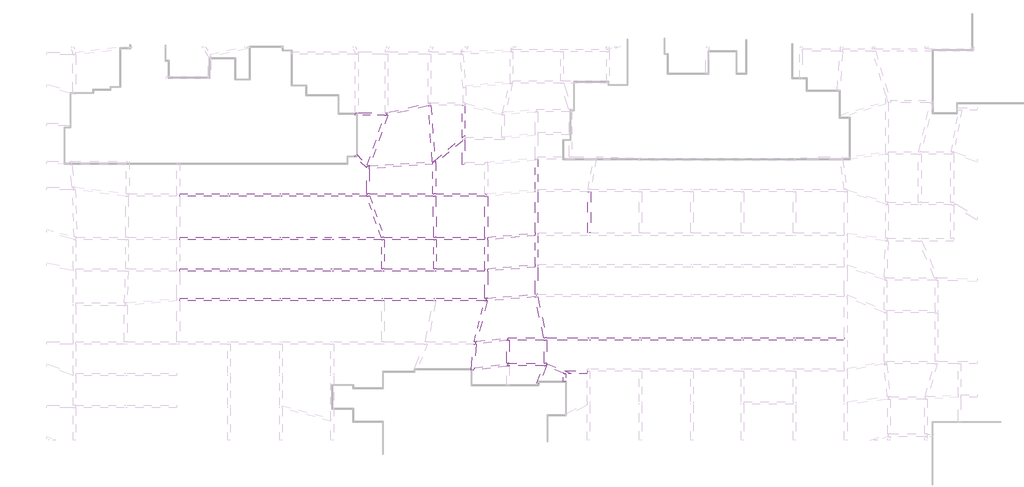
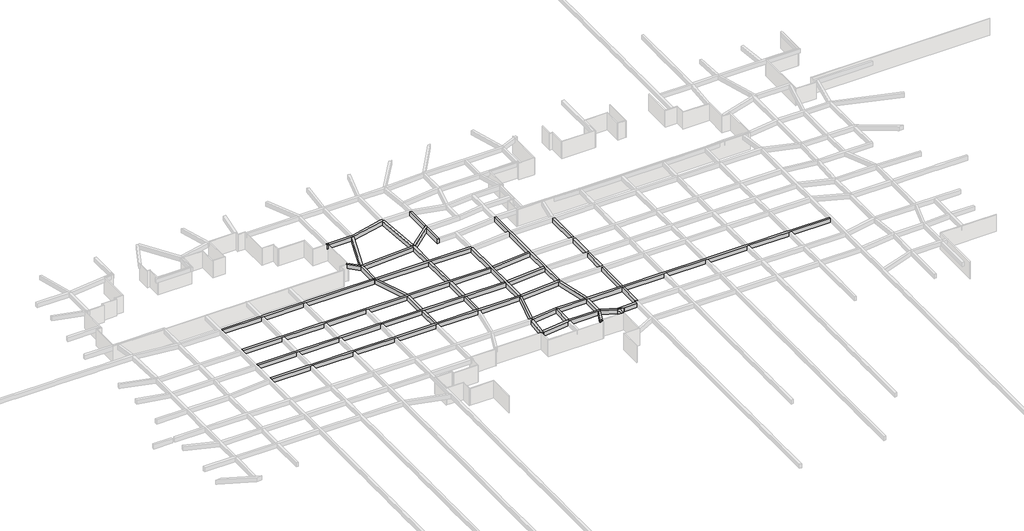
# One storey, part 29 of 45: 39 beams.
"""IFC4 building model written with IfcOpenShell, lengths in millimetres."""

import ifcopenshell
import ifcopenshell.guid

model = None  # the IFC model being written
_history = None  # IfcOwnerHistory: only IFC2X3 demands one
_inside = {}  # id of a spatial element -> (the spatial element, [elements in it])
_under = {}  # id of a project, library or spatial element -> (it, [spatial elements below it])
_declared = {}  # id of a project -> (the project, [libraries it declares])
_typed = {}  # id of a type object -> (the type object, [elements of that type])
_made_of = {}  # id of a material, layer set ... -> (it, [elements and type objects made of it])


def new_model(schema):
    """Start an empty IFC model of exactly this schema.

    Asked for "IFC4X3", IfcOpenShell would pick the latest addendum, in which some entities
    have other attributes; the version numbers below select the first issue.
    IFC2X3 requires an IfcOwnerHistory on every rooted entity: one is made here for all.
    """
    global model, _history
    if schema == "IFC4X3":
        model = ifcopenshell.file(schema_version=(4, 3, 0, 0))
    else:
        model = ifcopenshell.file(schema=schema)
    _inside.clear()
    _under.clear()
    _declared.clear()
    _typed.clear()
    _made_of.clear()
    _history = None
    if model.schema == "IFC2X3":
        org = make("IfcOrganization", Name="unknown")
        user = make(
            "IfcPersonAndOrganization",
            ThePerson=make("IfcPerson", FamilyName="unknown"),
            TheOrganization=org,
        )
        app = make(
            "IfcApplication",
            ApplicationDeveloper=org,
            Version="unknown",
            ApplicationFullName="unknown",
            ApplicationIdentifier="unknown",
        )
        _history = make(
            "IfcOwnerHistory",
            OwningUser=user,
            OwningApplication=app,
            ChangeAction="ADDED",
            CreationDate=0,
        )
    return model


def make(cls, **values):
    """One entity of the class cls with the attributes given. An attribute that is None is left unset."""
    return model.create_entity(
        cls, **{name: value for name, value in values.items() if value is not None}
    )


def rooted(cls, **values):
    """An entity with a GlobalId (a new one), such as an element, a storey or a relation."""
    return make(cls, GlobalId=ifcopenshell.guid.new(), OwnerHistory=_history, **values)


def si_unit(unit_type, name, prefix=None):
    """IfcSIUnit, for example si_unit("LENGTHUNIT", "METRE", prefix="MILLI")."""
    return make("IfcSIUnit", UnitType=unit_type, Prefix=prefix, Name=name)


def assignment(units):
    """IfcUnitAssignment: the units of a project."""
    return None if units is None else make("IfcUnitAssignment", Units=units)


def point(xyz):
    """IfcCartesianPoint."""
    return None if xyz is None else make("IfcCartesianPoint", Coordinates=xyz)


def direction(xyz):
    """IfcDirection."""
    return None if xyz is None else make("IfcDirection", DirectionRatios=xyz)


def frame(location, z_axis=None, x_axis=None):
    """IfcAxis2Placement3D, a coordinate frame: its origin and axes. An axis left out is left unset."""
    return make(
        "IfcAxis2Placement3D",
        Location=point(location),
        Axis=direction(z_axis),
        RefDirection=direction(x_axis),
    )


def origin():
    """The frame at (0, 0, 0) with its axes left unset."""
    return frame((0.0, 0.0, 0.0))


def place(relative_to, where):
    """IfcLocalPlacement: puts the frame where relative to a parent placement (None: the world)."""
    return make(
        "IfcLocalPlacement", PlacementRelTo=relative_to, RelativePlacement=where
    )


def context(
    kind, dimensions, precision=None, world=None, true_north=None, identifier=None
):
    """IfcGeometricRepresentationContext, for example the 3D "Model" context."""
    return make(
        "IfcGeometricRepresentationContext",
        ContextIdentifier=identifier,
        ContextType=kind,
        CoordinateSpaceDimension=dimensions,
        Precision=precision,
        WorldCoordinateSystem=world,
        TrueNorth=true_north,
    )


def project(units=None, contexts=None):
    """IfcProject with its units and contexts."""
    return rooted(
        "IfcProject",
        Name="project",
        RepresentationContexts=contexts,
        UnitsInContext=assignment(units),
    )


def spatial(cls, under=None, at=None, **own):
    """A site, building, storey or space (cls), placed at a placement, below another one or the project."""
    s = rooted(cls, ObjectPlacement=at, **own)
    if under is not None:
        _under.setdefault(under.id(), (under, []))[1].append(s)
    return s


def polyline(points):
    """IfcPolyline through the points."""
    return make("IfcPolyline", Points=[point(p) for p in points])


def outline(outer, holes=None, kind="AREA"):
    """IfcArbitraryClosedProfileDef: a profile drawn as a closed curve; with holes, ...WithVoids."""
    if holes is None:
        return make("IfcArbitraryClosedProfileDef", ProfileType=kind, OuterCurve=outer)
    return make(
        "IfcArbitraryProfileDefWithVoids",
        ProfileType=kind,
        OuterCurve=outer,
        InnerCurves=holes,
    )


def extrude(swept, where, along, depth):
    """IfcExtrudedAreaSolid: the profile swept, set in the frame where, extruded along a direction by depth."""
    return make(
        "IfcExtrudedAreaSolid",
        SweptArea=swept,
        Position=where,
        ExtrudedDirection=direction(along),
        Depth=depth,
    )


def faces_of(points, faces, orient=None, outer=None):
    """IfcFace entities. A face is a list of loops; a loop is a list of indices into points, from 0.

    orient and outer hold one flag for each loop. By default every Orientation is true, the
    first loop of a face is its IfcFaceOuterBound and the others are IfcFaceBound.
    """
    made = []
    for i, loops in enumerate(faces):
        bounds = []
        for j, loop in enumerate(loops):
            is_outer = j == 0 if outer is None else outer[i][j]
            bounds.append(
                make(
                    "IfcFaceOuterBound" if is_outer else "IfcFaceBound",
                    Bound=make("IfcPolyLoop", Polygon=[points[k] for k in loop]),
                    Orientation=True if orient is None else orient[i][j],
                )
            )
        made.append(make("IfcFace", Bounds=bounds))
    return made


def faceted_brep(points, faces, orient=None, outer=None, voids=None):
    """IfcFacetedBrep: a solid bounded by flat faces; with voids (closed shells), ...WithVoids."""
    shared = [point(p) for p in points]
    hull = make("IfcClosedShell", CfsFaces=faces_of(shared, faces, orient, outer))
    if voids is None:
        return make("IfcFacetedBrep", Outer=hull)
    return make(
        "IfcFacetedBrepWithVoids",
        Outer=hull,
        Voids=[
            make(cls, CfsFaces=faces_of(shared, fs, o, b)) for cls, fs, o, b in voids
        ],
    )


def shape(context_of_items, identifier, shape_type, items):
    """IfcShapeRepresentation: the items that make up one representation, for example the "Body"."""
    return make(
        "IfcShapeRepresentation",
        ContextOfItems=context_of_items,
        RepresentationIdentifier=identifier,
        RepresentationType=shape_type,
        Items=items,
    )


def made_of(thing, what):
    """Note that an element or type object is made of a material, layer set ...; save() writes the relation."""
    if what is not None:
        _made_of.setdefault(what.id(), (what, []))[1].append(thing)
    return thing


def element(
    cls,
    number,
    at=None,
    inside=None,
    cuts=None,
    type_object=None,
    material=None,
    context=None,
    identifier="Body",
    shape_type=None,
    held_by="IfcProductDefinitionShape",
    body=None,
    shapes=None,
    **own,
):
    """One element of the class cls, such as IfcWall. Its Tag is "e" and its number.

    at: its placement. inside: the storey or other place that contains it. cuts: it is an
    opening in that element (IfcRelVoidsElement). A single representation is given by context,
    identifier, shape_type and body (its items); several are given by shapes. held_by: the class
    of the entity that holds the representations. save() writes the other relations.
    """
    e = rooted(cls, Tag="e%d" % number, ObjectPlacement=at, **own)
    if body is not None:
        shapes = [shape(context, identifier, shape_type, body)]
    if shapes is not None:
        e.Representation = make(held_by, Representations=shapes)
    if inside is not None:
        _inside.setdefault(inside.id(), (inside, []))[1].append(e)
    if cuts is not None:
        rooted(
            "IfcRelVoidsElement", RelatingBuildingElement=cuts, RelatedOpeningElement=e
        )
    if type_object is not None:
        _typed.setdefault(type_object.id(), (type_object, []))[1].append(e)
    return made_of(e, material)


def aggregate(whole, parts):
    """IfcRelAggregates: a whole, such as a stair, and the parts it consists of."""
    return rooted("IfcRelAggregates", RelatingObject=whole, RelatedObjects=parts)


def save(model, path):
    """Write the relations noted so far, then the file.

    IfcRelAggregates (storeys below a building ...), IfcRelContainedInSpatialStructure (elements
    in a storey), IfcRelDefinesByType, IfcRelAssociatesMaterial and IfcRelDeclares: one each for
    every whole, place, type object, material and project.
    """
    for whole, parts in _under.values():
        aggregate(whole, parts)
    for where, things in _inside.values():
        rooted(
            "IfcRelContainedInSpatialStructure",
            RelatedElements=things,
            RelatingStructure=where,
        )
    for kind, things in _typed.values():
        rooted("IfcRelDefinesByType", RelatedObjects=things, RelatingType=kind)
    for what, things in _made_of.values():
        rooted("IfcRelAssociatesMaterial", RelatedObjects=things, RelatingMaterial=what)
    for by, libraries in _declared.values():
        rooted("IfcRelDeclares", RelatingContext=by, RelatedDefinitions=libraries)
    model.write(path)


model = new_model("IFC4")

# Units and contexts
model_context = context("Model", 3, world=origin())
ifc_project = project(units=[si_unit("LENGTHUNIT", "METRE", prefix="MILLI")], contexts=[model_context])

# Site, building, storey
site = spatial("IfcSite", under=ifc_project)
building = spatial("IfcBuilding", under=site)
storey = spatial("IfcBuildingStorey", under=building, Name="户型图", Elevation=0.0)

# Beams
placement = place(None, origin())
element("IfcBeam", 1, ObjectType="混凝土 - 矩形梁 : KL_beam", at=placement, inside=storey, context=model_context, shape_type="Brep", body=[
    faceted_brep([(-45052.7606684, 62754.9176978, 3300.0), (-45098.3349117, 63154.9176978, 3300.0), (-45307.1090692, 63154.9176978, 3300.0), (-49450.5494811, 63154.9176978, 3300.0), (-49850.5494811, 63154.9176978, 3300.0), (-49850.5494811, 62754.9176978, 3300.0), (-45389.7997082, 62754.9176978, 3300.0), (-45052.7606684, 62754.9176978, 2500.0), (-49850.5494811, 62754.9176978, 2500.0), (-45389.7997082, 62754.9176978, 2500.0), (-45098.3349117, 63154.9176978, 2500.0), (-49850.5494811, 63154.9176978, 2500.0), (-49450.5494811, 63154.9176978, 2500.0), (-45307.1090692, 63154.9176978, 2500.0)], [[[0, 1, 2, 3, 4, 5, 6]], [[7, 0, 6, 5, 8, 9]], [[10, 7, 9, 8, 11, 12, 13]], [[1, 10, 13, 12, 11, 4, 3, 2]], [[1, 0, 7, 10]], [[5, 4, 11, 8]]]),
])
element("IfcBeam", 2, ObjectType="混凝土 - 矩形梁 : KL_beam", at=placement, inside=storey, context=model_context, shape_type="Brep", body=[
    faceted_brep([(-38570.0554777, 64662.0897619, 3300.0), (-38787.1090692, 64611.9789919, 3300.0), (-44907.1090692, 63199.0656622, 3300.0), (-45098.3349117, 63154.9176978, 3300.0), (-45052.7606684, 62754.9176978, 3300.0), (-44957.8795294, 62776.8227348, 3300.0), (-38770.4179692, 64205.3107928, 3300.0), (-38524.4812344, 64262.0897619, 3300.0), (-45052.7606684, 62754.9176978, 2500.0), (-44957.8795294, 62776.8227348, 2500.0), (-38770.4179692, 64205.3107928, 2500.0), (-38524.4812344, 64262.0897619, 2500.0), (-45098.3349117, 63154.9176978, 2500.0), (-44907.1090692, 63199.0656622, 2500.0), (-38787.1090692, 64611.9789919, 2500.0), (-38570.0554777, 64662.0897619, 2500.0)], [[[0, 1, 2, 3, 4, 5, 6, 7]], [[7, 6, 5, 4, 8, 9, 10, 11]], [[11, 10, 9, 8, 12, 13, 14, 15]], [[3, 2, 1, 0, 15, 14, 13, 12]], [[3, 12, 8, 4]], [[0, 7, 11, 15]]]),
])
element("IfcBeam", 3, ObjectType="混凝土 - 矩形梁 : KL_beam", at=placement, inside=storey, context=model_context, shape_type="Brep", body=[
    faceted_brep([(-29959.2503222, 50450.070339, 3300.0), (-29976.7146993, 50850.070339, 3300.0), (-30167.9825107, 50850.070339, 3300.0), (-37667.9825107, 50850.070339, 3300.0), (-38067.9825107, 50850.070339, 3300.0), (-47767.9825107, 50850.070339, 3300.0), (-48167.9825107, 50850.070339, 3300.0), (-48167.9825107, 50450.070339, 3300.0), (-48110.2368931, 50450.070339, 3300.0), (-47686.7585782, 50450.070339, 3300.0), (-38064.5219634, 50450.070339, 3300.0), (-37664.4610322, 50450.070339, 3300.0), (-30167.9825107, 50450.070339, 3300.0), (-29959.2503222, 50450.070339, 2500.0), (-48167.9825107, 50450.070339, 2500.0), (-48110.2368931, 50450.070339, 2500.0), (-47686.7585782, 50450.070339, 2500.0), (-38064.5219634, 50450.070339, 2500.0), (-37664.4610322, 50450.070339, 2500.0), (-30167.9825107, 50450.070339, 2500.0), (-29976.7146993, 50850.070339, 2500.0), (-48167.9825107, 50850.070339, 2500.0), (-47767.9825107, 50850.070339, 2500.0), (-38067.9825107, 50850.070339, 2500.0), (-37667.9825107, 50850.070339, 2500.0), (-30167.9825107, 50850.070339, 2500.0)], [[[0, 1, 2, 3, 4, 5, 6, 7, 8, 9, 10, 11, 12]], [[13, 0, 12, 11, 10, 9, 8, 7, 14, 15, 16, 17, 18, 19]], [[20, 13, 19, 18, 17, 16, 15, 14, 21, 22, 23, 24, 25]], [[1, 20, 25, 24, 23, 22, 21, 6, 5, 4, 3, 2]], [[1, 0, 13, 20]], [[7, 6, 21, 14]]]),
])
element("IfcBeam", 4, ObjectType="混凝土 - 矩形梁 : KL_beam", at=placement, inside=storey, context=model_context, shape_type="Brep", body=[
    faceted_brep([(-37667.9825107, 55736.6887225, 3300.0), (-38067.9825107, 55736.6887225, 3300.0), (-38067.9825107, 55335.7291833, 3300.0), (-38067.9825107, 50850.070339, 3300.0), (-37667.9825107, 50850.070339, 3300.0), (-37667.9825107, 55456.8088074, 3300.0), (-37667.9825107, 55736.6887225, 2500.0), (-37667.9825107, 50850.070339, 2500.0), (-37667.9825107, 55456.8088074, 2500.0), (-38067.9825107, 55736.6887225, 2500.0), (-38067.9825107, 50850.070339, 2500.0), (-38067.9825107, 55335.7291833, 2500.0)], [[[0, 1, 2, 3, 4, 5]], [[6, 0, 5, 4, 7, 8]], [[9, 6, 8, 7, 10, 11]], [[1, 9, 11, 10, 3, 2]], [[4, 3, 10, 7]], [[1, 0, 6, 9]]]),
])
element("IfcBeam", 5, ObjectType="混凝土 - 矩形梁 : KL_beam", at=placement, inside=storey, context=model_context, shape_type="Brep", body=[
    faceted_brep([(-47767.9825107, 55064.4114948, 3300.0), (-47890.9579068, 55055.8884476, 3300.0), (-48167.9825107, 55036.6887225, 3300.0), (-48167.9825107, 54767.2276266, 3300.0), (-48167.9825107, 50850.070339, 3300.0), (-47767.9825107, 50850.070339, 3300.0), (-47767.9825107, 54663.4519556, 3300.0), (-47767.9825107, 55064.4114948, 2500.0), (-47767.9825107, 50850.070339, 2500.0), (-47767.9825107, 54663.4519556, 2500.0), (-48167.9825107, 55036.6887225, 2500.0), (-47890.9579068, 55055.8884476, 2500.0), (-48167.9825107, 50850.070339, 2500.0), (-48167.9825107, 54767.2276266, 2500.0)], [[[0, 1, 2, 3, 4, 5, 6]], [[7, 0, 6, 5, 8, 9]], [[10, 11, 7, 9, 8, 12, 13]], [[2, 10, 13, 12, 4, 3]], [[5, 4, 12, 8]], [[2, 1, 0, 7, 11, 10]]]),
])
element("IfcBeam", 6, ObjectType="混凝土 - 矩形梁 : KL_beam", at=placement, inside=storey, context=model_context, shape_type="Brep", body=[
    faceted_brep([(-37667.9825107, 55736.6887225, 3300.0), (-37667.9825107, 55764.4114948, 3300.0), (-37946.7071962, 55745.0939423, 3300.0), (-38067.9825107, 55736.6887225, 3300.0), (-38067.9825107, 55335.7291833, 2500.0), (-38067.9825107, 55335.7291833, 3300.0), (-47767.9825107, 54663.4519556, 3300.0), (-47767.9825107, 54663.4519556, 2500.0), (-37667.9825107, 55764.4114948, 2500.0), (-37667.9825107, 55736.6887225, 2500.0), (-38067.9825107, 55736.6887225, 2500.0), (-37946.7071962, 55745.0939423, 2500.0), (-38182.931614, 55728.721953, 2500.0), (-47678.0290506, 55070.645893, 2500.0), (-47767.9825107, 55064.4114948, 2500.0), (-47767.9825107, 55064.4114948, 3300.0), (-47678.0290506, 55070.645893, 3300.0), (-38182.931614, 55728.721953, 3300.0)], [[[0, 1, 2, 3]], [[4, 5, 6, 7]], [[8, 9, 10, 11]], [[1, 8, 11, 10, 12, 13, 14, 15, 16, 17, 3, 2]], [[8, 1, 0, 9]], [[10, 3, 5, 4]], [[3, 10, 9, 0]], [[5, 3, 17, 16, 15, 6]], [[10, 4, 7, 14, 13, 12]], [[7, 6, 15, 14]]]),
])
element("IfcBeam", 7, ObjectType="混凝土 - 矩形梁 : KL_beam", at=placement, inside=storey, context=model_context, shape_type="Brep", body=[
    faceted_brep([(-37667.9825107, 55764.4114948, 3300.0), (-37667.9825107, 55736.6887225, 3300.0), (-37667.9825107, 55456.8088074, 3300.0), (-33647.587215, 58830.3210173, 3300.0), (-33374.1168986, 59059.7898589, 3300.0), (-33247.268356, 59166.2284242, 3300.0), (-33247.268356, 59459.7898589, 3300.0), (-33247.268356, 59688.3913399, 3300.0), (-33647.268356, 59352.7514875, 3300.0), (-37792.0981227, 55874.8263589, 3300.0), (-37946.7071962, 55745.0939423, 3300.0), (-37667.9825107, 55456.8088074, 2500.0), (-33647.587215, 58830.3210173, 2500.0), (-33374.1168986, 59059.7898589, 2500.0), (-33247.268356, 59166.2284242, 2500.0), (-37667.9825107, 55736.6887225, 2500.0), (-37667.9825107, 55764.4114948, 2500.0), (-37946.7071962, 55745.0939423, 2500.0), (-37792.0981227, 55874.8263589, 2500.0), (-33647.268356, 59352.7514875, 2500.0), (-33247.268356, 59688.3913399, 2500.0), (-33247.268356, 59459.7898589, 2500.0)], [[[0, 1, 2, 3, 4, 5, 6, 7, 8, 9, 10]], [[2, 11, 12, 13, 14, 5, 4, 3]], [[11, 15, 16, 17, 18, 19, 20, 21, 14, 13, 12]], [[7, 20, 19, 18, 17, 10, 9, 8]], [[0, 16, 15, 11, 2, 1]], [[16, 0, 10, 17]], [[7, 6, 5, 14, 21, 20]]]),
])
element("IfcBeam", 8, ObjectType="混凝土 - 矩形梁 : KL_beam", at=placement, inside=storey, context=model_context, shape_type="Brep", body=[
    faceted_brep([(-33247.268356, 64262.0897619, 3300.0), (-33647.268356, 64262.0897619, 3300.0), (-33647.268356, 59352.7514875, 3300.0), (-33247.268356, 59688.3913399, 3300.0), (-33247.268356, 64205.7588739, 3300.0), (-33647.268356, 64262.0897619, 2500.0), (-33647.268356, 59352.7514875, 2500.0), (-33247.268356, 64262.0897619, 2500.0), (-33247.268356, 64205.7588739, 2500.0), (-33247.268356, 59688.3913399, 2500.0)], [[[0, 1, 2, 3, 4]], [[1, 5, 6, 2]], [[5, 7, 8, 9, 6]], [[7, 0, 4, 3, 9, 8]], [[1, 0, 7, 5]], [[3, 2, 6, 9]]]),
])
element("IfcBeam", 9, ObjectType="混凝土 - 矩形梁 : KL_beam", at=placement, inside=storey, context=model_context, shape_type="Brep", body=[
    faceted_brep([(-26695.4657952, 28984.9161885, 3300.0), (-26671.1423049, 28584.9161885, 3300.0), (-26483.2936927, 28584.9161885, 3300.0), (-21183.2936927, 28584.9161885, 3300.0), (-20783.2936927, 28584.9161885, 3300.0), (-14537.8475592, 28584.9161885, 3300.0), (-14137.8475592, 28584.9161885, 3300.0), (-6728.2347705, 28584.9161885, 3300.0), (-6328.2347705, 28584.9161885, 3300.0), (1071.7652295, 28584.9161885, 3300.0), (1471.7652295, 28584.9161885, 3300.0), (8769.3873949, 28584.9161885, 3300.0), (9169.3873949, 28584.9161885, 3300.0), (16669.3873949, 28584.9161885, 3300.0), (17069.3873949, 28584.9161885, 3300.0), (24442.7166646, 28584.9161885, 3300.0), (24442.7166646, 28984.9161885, 3300.0), (17069.3873949, 28984.9161885, 3300.0), (16669.3873949, 28984.9161885, 3300.0), (9169.3873949, 28984.9161885, 3300.0), (8769.3873949, 28984.9161885, 3300.0), (1471.7652295, 28984.9161885, 3300.0), (1071.7652295, 28984.9161885, 3300.0), (-6328.2347705, 28984.9161885, 3300.0), (-6728.2347705, 28984.9161885, 3300.0), (-14137.8475592, 28984.9161885, 3300.0), (-14537.8475592, 28984.9161885, 3300.0), (-20822.0981997, 28984.9161885, 3300.0), (-21231.4395884, 28984.9161885, 3300.0), (-26671.1423049, 28584.9161885, 2500.0), (-26483.2936927, 28584.9161885, 2500.0), (-21183.2936927, 28584.9161885, 2500.0), (-20783.2936927, 28584.9161885, 2500.0), (-14537.8475592, 28584.9161885, 2500.0), (-14137.8475592, 28584.9161885, 2500.0), (-6728.2347705, 28584.9161885, 2500.0), (-6328.2347705, 28584.9161885, 2500.0), (1071.7652295, 28584.9161885, 2500.0), (1471.7652295, 28584.9161885, 2500.0), (8769.3873949, 28584.9161885, 2500.0), (9169.3873949, 28584.9161885, 2500.0), (16669.3873949, 28584.9161885, 2500.0), (17069.3873949, 28584.9161885, 2500.0), (24442.7166646, 28584.9161885, 2500.0), (-26695.4657952, 28984.9161885, 2500.0), (-21231.4395884, 28984.9161885, 2500.0), (-20822.0981997, 28984.9161885, 2500.0), (-14537.8475592, 28984.9161885, 2500.0), (-14137.8475592, 28984.9161885, 2500.0), (-6728.2347705, 28984.9161885, 2500.0), (-6328.2347705, 28984.9161885, 2500.0), (1071.7652295, 28984.9161885, 2500.0), (1471.7652295, 28984.9161885, 2500.0), (8769.3873949, 28984.9161885, 2500.0), (9169.3873949, 28984.9161885, 2500.0), (16669.3873949, 28984.9161885, 2500.0), (17069.3873949, 28984.9161885, 2500.0), (24442.7166646, 28984.9161885, 2500.0)], [[[0, 1, 2, 3, 4, 5, 6, 7, 8, 9, 10, 11, 12, 13, 14, 15, 16, 17, 18, 19, 20, 21, 22, 23, 24, 25, 26, 27, 28]], [[1, 29, 30, 31, 32, 33, 34, 35, 36, 37, 38, 39, 40, 41, 42, 43, 15, 14, 13, 12, 11, 10, 9, 8, 7, 6, 5, 4, 3, 2]], [[29, 44, 45, 46, 47, 48, 49, 50, 51, 52, 53, 54, 55, 56, 57, 43, 42, 41, 40, 39, 38, 37, 36, 35, 34, 33, 32, 31, 30]], [[44, 0, 28, 27, 26, 25, 24, 23, 22, 21, 20, 19, 18, 17, 16, 57, 56, 55, 54, 53, 52, 51, 50, 49, 48, 47, 46, 45]], [[16, 15, 43, 57]], [[0, 44, 29, 1]]]),
])
element("IfcBeam", 10, ObjectType="混凝土 - 矩形梁 : KL_beam", at=placement, inside=storey, context=model_context, shape_type="Brep", body=[
    faceted_brep([(-29968.6853807, 34571.3370449, 3300.0), (-29984.5830666, 34971.3370449, 3300.0), (-30167.9825107, 34971.3370449, 3300.0), (-37583.2968796, 34971.3370449, 3300.0), (-37983.2968796, 34971.3370449, 3300.0), (-45471.0209029, 34971.3370449, 3300.0), (-45871.0209029, 34971.3370449, 3300.0), (-53171.0209029, 34971.3370449, 3300.0), (-53571.0209029, 34971.3370449, 3300.0), (-60985.2176693, 34971.3370449, 3300.0), (-61385.2176693, 34971.3370449, 3300.0), (-68859.410716, 34971.3370449, 3300.0), (-69259.410716, 34971.3370449, 3300.0), (-76574.0592951, 34971.3370449, 3300.0), (-76574.0592951, 34571.3370449, 3300.0), (-69259.410716, 34571.3370449, 3300.0), (-68859.410716, 34571.3370449, 3300.0), (-61385.2176693, 34571.3370449, 3300.0), (-60985.2176693, 34571.3370449, 3300.0), (-53571.0209029, 34571.3370449, 3300.0), (-53171.0209029, 34571.3370449, 3300.0), (-45871.0209029, 34571.3370449, 3300.0), (-45471.0209029, 34571.3370449, 3300.0), (-38025.9130936, 34571.3370449, 3300.0), (-37618.4264156, 34571.3370449, 3300.0), (-30235.0596889, 34571.3370449, 3300.0), (-29968.6853807, 34571.3370449, 2500.0), (-76574.0592951, 34571.3370449, 2500.0), (-69259.410716, 34571.3370449, 2500.0), (-68859.410716, 34571.3370449, 2500.0), (-61385.2176693, 34571.3370449, 2500.0), (-60985.2176693, 34571.3370449, 2500.0), (-53571.0209029, 34571.3370449, 2500.0), (-53171.0209029, 34571.3370449, 2500.0), (-45871.0209029, 34571.3370449, 2500.0), (-45471.0209029, 34571.3370449, 2500.0), (-38025.9130936, 34571.3370449, 2500.0), (-37618.4264156, 34571.3370449, 2500.0), (-30235.0596889, 34571.3370449, 2500.0), (-29984.5830666, 34971.3370449, 2500.0), (-76574.0592951, 34971.3370449, 2500.0), (-69259.410716, 34971.3370449, 2500.0), (-68859.410716, 34971.3370449, 2500.0), (-61385.2176693, 34971.3370449, 2500.0), (-60985.2176693, 34971.3370449, 2500.0), (-53571.0209029, 34971.3370449, 2500.0), (-53171.0209029, 34971.3370449, 2500.0), (-45871.0209029, 34971.3370449, 2500.0), (-45471.0209029, 34971.3370449, 2500.0), (-37983.2968796, 34971.3370449, 2500.0), (-37583.2968796, 34971.3370449, 2500.0), (-30167.9825107, 34971.3370449, 2500.0)], [[[0, 1, 2, 3, 4, 5, 6, 7, 8, 9, 10, 11, 12, 13, 14, 15, 16, 17, 18, 19, 20, 21, 22, 23, 24, 25]], [[26, 0, 25, 24, 23, 22, 21, 20, 19, 18, 17, 16, 15, 14, 27, 28, 29, 30, 31, 32, 33, 34, 35, 36, 37, 38]], [[39, 26, 38, 37, 36, 35, 34, 33, 32, 31, 30, 29, 28, 27, 40, 41, 42, 43, 44, 45, 46, 47, 48, 49, 50, 51]], [[1, 39, 51, 50, 49, 48, 47, 46, 45, 44, 43, 42, 41, 40, 13, 12, 11, 10, 9, 8, 7, 6, 5, 4, 3, 2]], [[14, 13, 40, 27]], [[1, 0, 26, 39]]]),
])
element("IfcBeam", 11, ObjectType="混凝土 - 矩形梁 : KL_beam", at=placement, inside=storey, context=model_context, shape_type="Brep", body=[
    faceted_brep([(-76574.0592951, 39470.5101546, 3300.0), (-76574.0592951, 39070.5101546, 3300.0), (-69259.410716, 39070.5101546, 3300.0), (-68859.410716, 39070.5101546, 3300.0), (-61385.2176693, 39070.5101546, 3300.0), (-60985.2176693, 39070.5101546, 3300.0), (-53571.0209029, 39070.5101546, 3300.0), (-53171.0209029, 39070.5101546, 3300.0), (-45871.0209029, 39070.5101546, 3300.0), (-45471.0209029, 39070.5101546, 3300.0), (-37983.2968796, 39070.5101546, 3300.0), (-37583.2968796, 39070.5101546, 3300.0), (-30167.9825107, 39070.5101546, 3300.0), (-30167.9825107, 39470.5101546, 3300.0), (-37583.2968796, 39470.5101546, 3300.0), (-37983.2968796, 39470.5101546, 3300.0), (-45471.0209029, 39470.5101546, 3300.0), (-45871.0209029, 39470.5101546, 3300.0), (-53171.0209029, 39470.5101546, 3300.0), (-53571.0209029, 39470.5101546, 3300.0), (-60985.2176693, 39470.5101546, 3300.0), (-61385.2176693, 39470.5101546, 3300.0), (-68859.410716, 39470.5101546, 3300.0), (-69259.410716, 39470.5101546, 3300.0), (-76574.0592951, 39070.5101546, 2500.0), (-69259.410716, 39070.5101546, 2500.0), (-68859.410716, 39070.5101546, 2500.0), (-61385.2176693, 39070.5101546, 2500.0), (-60985.2176693, 39070.5101546, 2500.0), (-53571.0209029, 39070.5101546, 2500.0), (-53171.0209029, 39070.5101546, 2500.0), (-45871.0209029, 39070.5101546, 2500.0), (-45471.0209029, 39070.5101546, 2500.0), (-37983.2968796, 39070.5101546, 2500.0), (-37583.2968796, 39070.5101546, 2500.0), (-30167.9825107, 39070.5101546, 2500.0), (-76574.0592951, 39470.5101546, 2500.0), (-69259.410716, 39470.5101546, 2500.0), (-68859.410716, 39470.5101546, 2500.0), (-61385.2176693, 39470.5101546, 2500.0), (-60985.2176693, 39470.5101546, 2500.0), (-53571.0209029, 39470.5101546, 2500.0), (-53171.0209029, 39470.5101546, 2500.0), (-45871.0209029, 39470.5101546, 2500.0), (-45471.0209029, 39470.5101546, 2500.0), (-37983.2968796, 39470.5101546, 2500.0), (-37583.2968796, 39470.5101546, 2500.0), (-30167.9825107, 39470.5101546, 2500.0)], [[[0, 1, 2, 3, 4, 5, 6, 7, 8, 9, 10, 11, 12, 13, 14, 15, 16, 17, 18, 19, 20, 21, 22, 23]], [[1, 24, 25, 26, 27, 28, 29, 30, 31, 32, 33, 34, 35, 12, 11, 10, 9, 8, 7, 6, 5, 4, 3, 2]], [[24, 36, 37, 38, 39, 40, 41, 42, 43, 44, 45, 46, 47, 35, 34, 33, 32, 31, 30, 29, 28, 27, 26, 25]], [[36, 0, 23, 22, 21, 20, 19, 18, 17, 16, 15, 14, 13, 47, 46, 45, 44, 43, 42, 41, 40, 39, 38, 37]], [[1, 0, 36, 24]], [[13, 12, 35, 47]]]),
])
element("IfcBeam", 12, ObjectType="混凝土 - 矩形梁 : KL_beam", at=placement, inside=storey, context=model_context, shape_type="Brep", body=[
    faceted_brep([(-76574.0592951, 44242.2010773, 3300.0), (-76574.0592951, 43842.2010773, 3300.0), (-69259.410716, 43842.2010773, 3300.0), (-68859.410716, 43842.2010773, 3300.0), (-61385.2176693, 43842.2010773, 3300.0), (-60985.2176693, 43842.2010773, 3300.0), (-53571.0209029, 43842.2010773, 3300.0), (-53171.0209029, 43842.2010773, 3300.0), (-45871.0209029, 43842.2010773, 3300.0), (-45471.0209029, 43842.2010773, 3300.0), (-37983.2968796, 43842.2010773, 3300.0), (-37583.2968796, 43842.2010773, 3300.0), (-30167.9825107, 43842.2010773, 3300.0), (-30167.9825107, 44242.2010773, 3300.0), (-37556.1022711, 44242.2010773, 3300.0), (-37956.1632023, 44242.2010773, 3300.0), (-45528.8049128, 44242.2010773, 3300.0), (-45952.2832276, 44242.2010773, 3300.0), (-60985.2176693, 44242.2010773, 3300.0), (-61385.2176693, 44242.2010773, 3300.0), (-68859.410716, 44242.2010773, 3300.0), (-69259.410716, 44242.2010773, 3300.0), (-76574.0592951, 43842.2010773, 2500.0), (-69259.410716, 43842.2010773, 2500.0), (-68859.410716, 43842.2010773, 2500.0), (-61385.2176693, 43842.2010773, 2500.0), (-60985.2176693, 43842.2010773, 2500.0), (-53571.0209029, 43842.2010773, 2500.0), (-53171.0209029, 43842.2010773, 2500.0), (-45871.0209029, 43842.2010773, 2500.0), (-45471.0209029, 43842.2010773, 2500.0), (-37983.2968796, 43842.2010773, 2500.0), (-37583.2968796, 43842.2010773, 2500.0), (-30167.9825107, 43842.2010773, 2500.0), (-76574.0592951, 44242.2010773, 2500.0), (-69259.410716, 44242.2010773, 2500.0), (-68859.410716, 44242.2010773, 2500.0), (-61385.2176693, 44242.2010773, 2500.0), (-60985.2176693, 44242.2010773, 2500.0), (-45952.2832276, 44242.2010773, 2500.0), (-45528.8049128, 44242.2010773, 2500.0), (-37956.1632023, 44242.2010773, 2500.0), (-37556.1022711, 44242.2010773, 2500.0), (-30167.9825107, 44242.2010773, 2500.0)], [[[0, 1, 2, 3, 4, 5, 6, 7, 8, 9, 10, 11, 12, 13, 14, 15, 16, 17, 18, 19, 20, 21]], [[1, 22, 23, 24, 25, 26, 27, 28, 29, 30, 31, 32, 33, 12, 11, 10, 9, 8, 7, 6, 5, 4, 3, 2]], [[22, 34, 35, 36, 37, 38, 39, 40, 41, 42, 43, 33, 32, 31, 30, 29, 28, 27, 26, 25, 24, 23]], [[34, 0, 21, 20, 19, 18, 17, 16, 15, 14, 13, 43, 42, 41, 40, 39, 38, 37, 36, 35]], [[1, 0, 34, 22]], [[13, 12, 33, 43]]]),
])
element("IfcBeam", 13, ObjectType="混凝土 - 矩形梁 : KL_beam", at=placement, inside=storey, context=model_context, shape_type="Brep", body=[
    faceted_brep([(-48167.9825107, 50450.070339, 3300.0), (-48167.9825107, 50850.070339, 3300.0), (-60985.2176693, 50850.070339, 3300.0), (-61385.2176693, 50850.070339, 3300.0), (-68859.410716, 50850.070339, 3300.0), (-69259.410716, 50850.070339, 3300.0), (-76574.0592951, 50850.070339, 3300.0), (-76574.0592951, 50450.070339, 3300.0), (-69259.410716, 50450.070339, 3300.0), (-68859.410716, 50450.070339, 3300.0), (-61385.2176693, 50450.070339, 3300.0), (-60985.2176693, 50450.070339, 3300.0), (-48167.9825107, 50450.070339, 2500.0), (-76574.0592951, 50450.070339, 2500.0), (-69259.410716, 50450.070339, 2500.0), (-68859.410716, 50450.070339, 2500.0), (-61385.2176693, 50450.070339, 2500.0), (-60985.2176693, 50450.070339, 2500.0), (-48167.9825107, 50850.070339, 2500.0), (-76574.0592951, 50850.070339, 2500.0), (-69259.410716, 50850.070339, 2500.0), (-68859.410716, 50850.070339, 2500.0), (-61385.2176693, 50850.070339, 2500.0), (-60985.2176693, 50850.070339, 2500.0)], [[[0, 1, 2, 3, 4, 5, 6, 7, 8, 9, 10, 11]], [[12, 0, 11, 10, 9, 8, 7, 13, 14, 15, 16, 17]], [[18, 12, 17, 16, 15, 14, 13, 19, 20, 21, 22, 23]], [[1, 18, 23, 22, 21, 20, 19, 6, 5, 4, 3, 2]], [[1, 0, 12, 18]], [[7, 6, 19, 13]]]),
])
element("IfcBeam", 14, ObjectType="混凝土 - 矩形梁 : KL_beam", at=placement, inside=storey, context=model_context, shape_type="SweptSolid", body=[
    extrude(outline(polyline([(-29767.9825107, 43858.9382014), (-29767.9825107, 44260.4661364), (-22564.0859234, 44890.725421), (-22564.0859234, 44489.197486), (-29767.9825107, 43858.9382014)])), frame((0.0, 0.0, 2500.0), z_axis=(0.0, 0.0, 1.0), x_axis=(1.0, 0.0, 0.0)), (0.0, 0.0, 1.0), 800.0),
])
element("IfcBeam", 15, ObjectType="混凝土 - 矩形梁 : KL_beam", at=placement, inside=storey, context=model_context, shape_type="SweptSolid", body=[
    extrude(outline(polyline([(-29767.9825107, 39086.539186), (-29767.9825107, 39487.9357642), (-22564.0859234, 40090.4451984), (-22564.0859234, 39689.0486202), (-29767.9825107, 39086.539186)])), frame((0.0, 0.0, 2500.0), z_axis=(0.0, 0.0, 1.0), x_axis=(1.0, 0.0, 0.0)), (0.0, 0.0, 1.0), 800.0),
])
element("IfcBeam", 16, ObjectType="混凝土 - 矩形梁 : KL_beam", at=placement, inside=storey, context=model_context, shape_type="Brep", body=[
    faceted_brep([(-22423.5665565, 35573.301237, 3300.0), (-22564.0859234, 35562.1139016, 3300.0), (-29767.9825107, 34988.5815224, 3300.0), (-29984.5830666, 34971.3370449, 3300.0), (-29968.6853807, 34571.3370449, 3300.0), (-29818.757949, 34583.2733957, 3300.0), (-22573.7714114, 35160.077118, 3300.0), (-22407.6688706, 35173.301237, 3300.0), (-29968.6853807, 34571.3370449, 2500.0), (-29818.757949, 34583.2733957, 2500.0), (-22573.7714114, 35160.077118, 2500.0), (-22407.6688706, 35173.301237, 2500.0), (-29984.5830666, 34971.3370449, 2500.0), (-29767.9825107, 34988.5815224, 2500.0), (-22564.0859234, 35562.1139016, 2500.0), (-22423.5665565, 35573.301237, 2500.0)], [[[0, 1, 2, 3, 4, 5, 6, 7]], [[7, 6, 5, 4, 8, 9, 10, 11]], [[11, 10, 9, 8, 12, 13, 14, 15]], [[3, 2, 1, 0, 15, 14, 13, 12]], [[0, 7, 11, 15]], [[3, 12, 8, 4]]]),
])
element("IfcBeam", 17, ObjectType="混凝土 - 矩形梁 : KL_beam", at=placement, inside=storey, context=model_context, shape_type="Brep", body=[
    faceted_brep([(-26695.4657952, 28984.9161885, 3300.0), (-31418.7094255, 28408.3553852, 3300.0), (-31613.4317995, 28384.5858537, 3300.0), (-31589.1083091, 27984.5858537, 3300.0), (-31499.1278227, 27995.569666, 3300.0), (-26883.2936927, 28559.0191177, 3300.0), (-26671.1423049, 28584.9161885, 3300.0), (-31589.1083091, 27984.5858537, 2500.0), (-31499.1278227, 27995.569666, 2500.0), (-26883.2936927, 28559.0191177, 2500.0), (-26671.1423049, 28584.9161885, 2500.0), (-31613.4317995, 28384.5858537, 2500.0), (-31418.7094255, 28408.3553852, 2500.0), (-26695.4657952, 28984.9161885, 2500.0)], [[[0, 1, 2, 3, 4, 5, 6]], [[6, 5, 4, 3, 7, 8, 9, 10]], [[10, 9, 8, 7, 11, 12, 13]], [[2, 1, 0, 13, 12, 11]], [[0, 6, 10, 13]], [[2, 11, 7, 3]]]),
])
element("IfcBeam", 18, ObjectType="混凝土 - 矩形梁 : KL_beam", at=placement, inside=storey, context=model_context, shape_type="SweptSolid", body=[
    extrude(outline(polyline([(-26483.2936927, 25091.3386729), (-26883.2936927, 25091.3386729), (-26883.2936927, 28559.0191177), (-26671.1423049, 28584.9161885), (-26483.2936927, 28584.9161885), (-26483.2936927, 25091.3386729)])), frame((0.0, 0.0, 2500.0), z_axis=(0.0, 0.0, 1.0), x_axis=(1.0, 0.0, 0.0)), (0.0, 0.0, 1.0), 800.0),
])
element("IfcBeam", 19, ObjectType="混凝土 - 矩形梁 : KL_beam", at=placement, inside=storey, context=model_context, shape_type="Brep", body=[
    faceted_brep([(-26683.2936927, 25084.9161885, 3300.0), (-26683.2936927, 25084.9161885, 2500.0), (-26683.2936927, 25053.8457271, 2500.0), (-26683.2936927, 24684.9161885, 2500.0), (-26683.2936927, 24684.9161885, 3300.0), (-26683.2936927, 25053.8457271, 3300.0), (-26404.4378825, 24684.9161885, 3300.0), (-21279.8058864, 24684.9161885, 3300.0), (-20848.3919894, 24684.9161885, 3300.0), (-20783.2936927, 24684.9161885, 3300.0), (-20783.2936927, 24846.0401267, 3300.0), (-20783.2936927, 25019.8178919, 3300.0), (-20783.2936927, 25084.9161885, 3300.0), (-21183.2936927, 25084.9161885, 3300.0), (-26404.4378825, 24684.9161885, 2500.0), (-21279.8058864, 24684.9161885, 2500.0), (-20848.3919894, 24684.9161885, 2500.0), (-20783.2936927, 24684.9161885, 2500.0), (-21183.2936927, 25084.9161885, 2500.0), (-20783.2936927, 25084.9161885, 2500.0), (-20783.2936927, 25019.8178919, 2500.0), (-20783.2936927, 24846.0401267, 2500.0)], [[[0, 1, 2, 3, 4, 5]], [[0, 5, 4, 6, 7, 8, 9, 10, 11, 12, 13]], [[4, 3, 14, 15, 16, 17, 9, 8, 7, 6]], [[3, 2, 1, 18, 19, 20, 21, 17, 16, 15, 14]], [[1, 0, 13, 12, 19, 18]], [[12, 11, 10, 9, 17, 21, 20, 19]]]),
])
element("IfcBeam", 20, ObjectType="混凝土 - 矩形梁 : KL_beam", at=placement, inside=storey, context=model_context, shape_type="SweptSolid", body=[
    extrude(outline(polyline([(-20783.2936927, 25084.9161885), (-21183.2936927, 25084.9161885), (-21183.2936927, 28584.9161885), (-20783.2936927, 28584.9161885), (-20783.2936927, 25084.9161885)])), frame((0.0, 0.0, 2500.0), z_axis=(0.0, 0.0, 1.0), x_axis=(1.0, 0.0, 0.0)), (0.0, 0.0, 1.0), 800.0),
])
element("IfcBeam", 21, ObjectType="混凝土 - 矩形梁 : KL_beam", at=placement, inside=storey, context=model_context, shape_type="SweptSolid", body=[
    extrude(outline(polyline([(-30235.0596889, 34571.3370449), (-29968.6853807, 34571.3370449), (-29818.757949, 34583.2733957), (-31418.7094255, 28408.3553852), (-31613.4317995, 28384.5858537), (-31838.0772004, 28384.5858537), (-30235.0596889, 34571.3370449)])), frame((0.0, 0.0, 2500.0), z_axis=(0.0, 0.0, 1.0), x_axis=(1.0, 0.0, 0.0)), (0.0, 0.0, 1.0), 800.0),
])
element("IfcBeam", 22, ObjectType="混凝土 - 矩形梁 : KL_beam", at=placement, inside=storey, context=model_context, shape_type="SweptSolid", body=[
    extrude(outline(polyline([(-45471.0209029, 34971.3370449), (-45871.0209029, 34971.3370449), (-45871.0209029, 39070.5101546), (-45471.0209029, 39070.5101546), (-45471.0209029, 34971.3370449)])), frame((0.0, 0.0, 2500.0), z_axis=(0.0, 0.0, 1.0), x_axis=(1.0, 0.0, 0.0)), (0.0, 0.0, 1.0), 800.0),
    extrude(outline(polyline([(-45871.0209029, 43842.2010773), (-45471.0209029, 43842.2010773), (-45471.0209029, 39470.5101546), (-45871.0209029, 39470.5101546), (-45871.0209029, 43842.2010773)])), frame((0.0, 0.0, 2500.0), z_axis=(0.0, 0.0, 1.0), x_axis=(1.0, 0.0, 0.0)), (0.0, 0.0, 1.0), 800.0),
])
element("IfcBeam", 23, ObjectType="混凝土 - 矩形梁 : KL_beam", at=placement, inside=storey, context=model_context, shape_type="SweptSolid", body=[
    extrude(outline(polyline([(-45528.8049128, 44242.2010773), (-45952.2832276, 44242.2010773), (-48110.2368931, 50450.070339), (-47686.7585782, 50450.070339), (-45528.8049128, 44242.2010773)])), frame((0.0, 0.0, 2500.0), z_axis=(0.0, 0.0, 1.0), x_axis=(1.0, 0.0, 0.0)), (0.0, 0.0, 1.0), 800.0),
])
element("IfcBeam", 24, ObjectType="混凝土 - 矩形梁 : KL_beam", at=placement, inside=storey, context=model_context, shape_type="SweptSolid", body=[
    extrude(outline(polyline([(-38064.5219634, 50450.070339), (-37664.4610322, 50450.070339), (-37556.1022711, 44242.2010773), (-37956.1632023, 44242.2010773), (-38064.5219634, 50450.070339)])), frame((0.0, 0.0, 2500.0), z_axis=(0.0, 0.0, 1.0), x_axis=(1.0, 0.0, 0.0)), (0.0, 0.0, 1.0), 800.0),
])
element("IfcBeam", 25, ObjectType="混凝土 - 矩形梁 : KL_beam", at=placement, inside=storey, context=model_context, shape_type="Brep", body=[
    faceted_brep([(-29959.2503222, 50450.070339, 3300.0), (-30167.9825107, 50450.070339, 3300.0), (-30167.9825107, 44242.2010773, 3300.0), (-30167.9825107, 43842.2010773, 3300.0), (-30167.9825107, 39470.5101546, 3300.0), (-30167.9825107, 39070.5101546, 3300.0), (-30167.9825107, 34971.3370449, 3300.0), (-30131.4177313, 34971.3370449, 3300.0), (-29984.5830666, 34971.3370449, 3300.0), (-29767.9825107, 34988.5815224, 3300.0), (-29767.9825107, 39086.539186, 3300.0), (-29767.9825107, 39487.9357642, 3300.0), (-29767.9825107, 43858.9382014, 3300.0), (-29767.9825107, 44260.4661364, 3300.0), (-29767.9825107, 50466.8041042, 3300.0), (-30167.9825107, 50450.070339, 2500.0), (-30167.9825107, 44242.2010773, 2500.0), (-30167.9825107, 43842.2010773, 2500.0), (-30167.9825107, 39470.5101546, 2500.0), (-30167.9825107, 39070.5101546, 2500.0), (-30167.9825107, 34971.3370449, 2500.0), (-29959.2503222, 50450.070339, 2500.0), (-29767.9825107, 50466.8041042, 2500.0), (-29767.9825107, 44260.4661364, 2500.0), (-29767.9825107, 43858.9382014, 2500.0), (-29767.9825107, 39487.9357642, 2500.0), (-29767.9825107, 39086.539186, 2500.0), (-29767.9825107, 34988.5815224, 2500.0), (-29984.5830666, 34971.3370449, 2500.0), (-30131.4177313, 34971.3370449, 2500.0)], [[[0, 1, 2, 3, 4, 5, 6, 7, 8, 9, 10, 11, 12, 13, 14]], [[1, 15, 16, 17, 18, 19, 20, 6, 5, 4, 3, 2]], [[15, 21, 22, 23, 24, 25, 26, 27, 28, 29, 20, 19, 18, 17, 16]], [[22, 14, 13, 12, 11, 10, 9, 27, 26, 25, 24, 23]], [[1, 0, 21, 15]], [[0, 14, 22, 21]], [[9, 8, 28, 27]], [[6, 20, 29, 28, 8, 7]]]),
])
element("IfcBeam", 26, ObjectType="混凝土 - 矩形梁 : KL_beam", at=placement, inside=storey, context=model_context, shape_type="SweptSolid", body=[
    extrude(outline(polyline([(-37583.2968796, 34971.3370449), (-37983.2968796, 34971.3370449), (-37983.2968796, 39070.5101546), (-37583.2968796, 39070.5101546), (-37583.2968796, 34971.3370449)])), frame((0.0, 0.0, 2500.0), z_axis=(0.0, 0.0, 1.0), x_axis=(1.0, 0.0, 0.0)), (0.0, 0.0, 1.0), 800.0),
    extrude(outline(polyline([(-37983.2968796, 43842.2010773), (-37583.2968796, 43842.2010773), (-37583.2968796, 39470.5101546), (-37983.2968796, 39470.5101546), (-37983.2968796, 43842.2010773)])), frame((0.0, 0.0, 2500.0), z_axis=(0.0, 0.0, 1.0), x_axis=(1.0, 0.0, 0.0)), (0.0, 0.0, 1.0), 800.0),
])
element("IfcBeam", 27, ObjectType="混凝土 - 矩形梁 : KL_beam", at=placement, inside=storey, context=model_context, shape_type="Brep", body=[
    faceted_brep([(-49947.8814981, 56547.1266139, 3300.0), (-49665.0387856, 56829.9693264, 3300.0), (-49665.0387856, 56829.9693264, 2500.0), (-49947.8814981, 56547.1266139, 2500.0), (-48167.9825107, 54767.2276266, 3300.0), (-48167.9825107, 55036.6887225, 3300.0), (-47890.9579068, 55055.8884476, 3300.0), (-48050.9513008, 55215.8818416, 3300.0), (-47890.9579068, 55055.8884476, 2500.0), (-48050.9513008, 55215.8818416, 2500.0), (-48167.9825107, 55036.6887225, 2500.0), (-48167.9825107, 54767.2276266, 2500.0)], [[[0, 1, 2, 3]], [[1, 0, 4, 5, 6, 7]], [[2, 1, 7, 6, 8, 9]], [[3, 2, 9, 8, 10, 11]], [[0, 3, 11, 4]], [[10, 5, 4, 11]], [[5, 10, 8, 6]]]),
])
element("IfcBeam", 28, ObjectType="混凝土 - 矩形梁 : KL_beam", at=placement, inside=storey, context=model_context, shape_type="Brep", body=[
    faceted_brep([(-38770.4179692, 64205.3107928, 3300.0), (-38182.931614, 55728.721953, 3300.0), (-38067.9825107, 55736.6887225, 3300.0), (-37946.7071962, 55745.0939423, 3300.0), (-37792.0981227, 55874.8263589, 3300.0), (-38373.3936061, 64262.0897619, 3300.0), (-38387.1090692, 64262.0897619, 3300.0), (-38524.4812344, 64262.0897619, 3300.0), (-38182.931614, 55728.721953, 2500.0), (-38770.4179692, 64205.3107928, 2500.0), (-38524.4812344, 64262.0897619, 2500.0), (-38387.1090692, 64262.0897619, 2500.0), (-38373.3936061, 64262.0897619, 2500.0), (-37792.0981227, 55874.8263589, 2500.0), (-37946.7071962, 55745.0939423, 2500.0), (-38067.9825107, 55736.6887225, 2500.0)], [[[0, 1, 2, 3, 4, 5, 6, 7]], [[8, 1, 0, 9]], [[8, 9, 10, 11, 12, 13, 14, 15]], [[12, 5, 4, 13]], [[1, 8, 15, 14, 3, 2]], [[0, 7, 10, 9]], [[5, 12, 11, 10, 7, 6]], [[4, 3, 14, 13]]]),
])
element("IfcBeam", 29, ObjectType="混凝土 - 矩形梁 : KL_beam", at=placement, inside=storey, context=model_context, shape_type="Brep", body=[
    faceted_brep([(-47678.0290506, 55070.645893, 3300.0), (-47678.0290506, 55070.645893, 2500.0), (-44957.8795294, 62776.8227348, 2500.0), (-44957.8795294, 62776.8227348, 3300.0), (-47767.9825107, 55064.4114948, 3300.0), (-47890.9579068, 55055.8884476, 3300.0), (-47890.9579068, 55055.8884476, 2500.0), (-47767.9825107, 55064.4114948, 2500.0), (-45052.7606684, 62754.9176978, 3300.0), (-45307.1090692, 62754.9176978, 3300.0), (-45389.7997082, 62754.9176978, 3300.0), (-48050.9513008, 55215.8818416, 3300.0), (-48050.9513008, 55215.8818416, 2500.0), (-45389.7997082, 62754.9176978, 2500.0), (-45307.1090692, 62754.9176978, 2500.0), (-45052.7606684, 62754.9176978, 2500.0)], [[[0, 1, 2, 3]], [[1, 0, 4, 5, 6, 7]], [[5, 4, 0, 3, 8, 9, 10, 11]], [[12, 11, 10, 13]], [[1, 7, 6, 12, 13, 14, 15, 2]], [[6, 5, 11, 12]], [[13, 10, 9, 8, 15, 14]], [[3, 2, 15, 8]]]),
])
element("IfcBeam", 30, ObjectType="混凝土 - 矩形梁 : KL_beam", at=placement, inside=storey, context=model_context, shape_type="Brep", body=[
    faceted_brep([(-31901.6167168, 27984.5858537, 3300.0), (-32245.3738344, 24055.4240199, 3300.0), (-31846.8959551, 24020.5617228, 3300.0), (-31811.2601461, 24427.8808841, 3300.0), (-31499.1278227, 27995.569666, 3300.0), (-31526.5309488, 27992.2245986, 3300.0), (-31589.1083091, 27984.5858537, 3300.0), (-31901.6167168, 27984.5858537, 2500.0), (-32245.3738344, 24055.4240199, 2500.0), (-31589.1083091, 27984.5858537, 2500.0), (-31526.5309488, 27992.2245986, 2500.0), (-31499.1278227, 27995.569666, 2500.0), (-31811.2601461, 24427.8808841, 2500.0), (-31846.8959551, 24020.5617228, 2500.0)], [[[0, 1, 2, 3, 4, 5, 6]], [[1, 0, 7, 8]], [[8, 7, 9, 10, 11, 12, 13]], [[4, 3, 2, 13, 12, 11]], [[0, 6, 9, 7]], [[4, 11, 10, 9, 6, 5]], [[2, 1, 8, 13]]]),
])
element("IfcBeam", 31, ObjectType="混凝土 - 矩形梁 : KL_beam", at=placement, inside=storey, context=model_context, shape_type="Brep", body=[
    faceted_brep([(-31811.2601461, 24427.8808841, 3300.0), (-31846.8959551, 24020.5617228, 3300.0), (-26883.2936927, 24626.4628221, 3300.0), (-26483.2936927, 24675.2903524, 3300.0), (-26404.4378825, 24684.9161885, 3300.0), (-26683.2936927, 24684.9161885, 3300.0), (-26683.2936927, 25053.8457271, 3300.0), (-31846.8959551, 24020.5617228, 2500.0), (-26883.2936927, 24626.4628221, 2500.0), (-26483.2936927, 24675.2903524, 2500.0), (-26404.4378825, 24684.9161885, 2500.0), (-31811.2601461, 24427.8808841, 2500.0), (-26683.2936927, 25053.8457271, 2500.0), (-26683.2936927, 24684.9161885, 2500.0)], [[[0, 1, 2, 3, 4, 5, 6]], [[1, 7, 8, 9, 10, 4, 3, 2]], [[7, 11, 12, 13, 10, 9, 8]], [[11, 0, 6, 12]], [[1, 0, 11, 7]], [[13, 5, 4, 10]], [[5, 13, 12, 6]]]),
])
element("IfcBeam", 32, ObjectType="混凝土 - 矩形梁 : KL_beam", at=placement, inside=storey, context=model_context, shape_type="Brep", body=[
    faceted_brep([(-21959.1373614, 21935.7249207, 3300.0), (-22330.0109032, 22085.5675581, 3300.0), (-22330.0109032, 22085.5675581, 2500.0), (-21959.1373614, 21935.7249207, 2500.0), (-20872.7782405, 24624.5580989, 3300.0), (-20848.3919894, 24684.9161885, 3300.0), (-21183.2936927, 24684.9161885, 3300.0), (-21279.8058864, 24684.9161885, 3300.0), (-21279.8058864, 24684.9161885, 2500.0), (-21183.2936927, 24684.9161885, 2500.0), (-20848.3919894, 24684.9161885, 2500.0), (-20872.7782405, 24624.5580989, 2500.0)], [[[0, 1, 2, 3]], [[1, 0, 4, 5, 6, 7]], [[2, 1, 7, 8]], [[3, 2, 8, 9, 10, 11]], [[0, 3, 11, 10, 5, 4]], [[8, 7, 6, 5, 10, 9]]]),
    faceted_brep([(-20722.9356031, 24995.4316408, 3300.0), (-20722.9356031, 24995.4316408, 2500.0), (-20783.2936927, 25019.8178919, 2500.0), (-20783.2936927, 25019.8178919, 3300.0), (-20783.2936927, 24846.0401267, 3300.0), (-20783.2936927, 24846.0401267, 2500.0)], [[[0, 1, 2, 3]], [[4, 3, 2, 5]], [[3, 4, 0]], [[5, 2, 1]], [[1, 0, 4, 5]]]),
])
element("IfcBeam", 33, ObjectType="混凝土 - 矩形梁 : KL_beam", at=placement, inside=storey, context=model_context, shape_type="Brep", body=[
    faceted_brep([(-22423.5665565, 35573.301237, 3300.0), (-22164.0859234, 35573.301237, 3300.0), (-22164.0859234, 39701.2747355, 3300.0), (-22164.0859234, 40101.2747355, 3300.0), (-22164.0859234, 44499.769125, 3300.0), (-22164.0859234, 44899.769125, 3300.0), (-22164.0859234, 51121.1695582, 3300.0), (-22164.0859234, 51521.1695582, 3300.0), (-22164.0859234, 56076.5180379, 3300.0), (-22564.0859234, 56076.5180379, 3300.0), (-22564.0859234, 55897.0633889, 3300.0), (-22564.0859234, 51498.5913239, 3300.0), (-22564.0859234, 51097.0633889, 3300.0), (-22564.0859234, 44890.725421, 3300.0), (-22564.0859234, 44489.197486, 3300.0), (-22564.0859234, 40090.4451984, 3300.0), (-22564.0859234, 39689.0486202, 3300.0), (-22564.0859234, 35562.1139016, 3300.0), (-22564.0859234, 56076.5180379, 2500.0), (-22564.0859234, 55897.0633889, 2500.0), (-22564.0859234, 51498.5913239, 2500.0), (-22564.0859234, 51097.0633889, 2500.0), (-22564.0859234, 44890.725421, 2500.0), (-22564.0859234, 44489.197486, 2500.0), (-22564.0859234, 40090.4451984, 2500.0), (-22564.0859234, 39689.0486202, 2500.0), (-22564.0859234, 35562.1139016, 2500.0), (-22164.0859234, 35573.301237, 2500.0), (-22423.5665565, 35573.301237, 2500.0), (-22164.0859234, 56076.5180379, 2500.0), (-22164.0859234, 51521.1695582, 2500.0), (-22164.0859234, 51121.1695582, 2500.0), (-22164.0859234, 44899.769125, 2500.0), (-22164.0859234, 44499.769125, 2500.0), (-22164.0859234, 40101.2747355, 2500.0), (-22164.0859234, 39701.2747355, 2500.0)], [[[0, 1, 2, 3, 4, 5, 6, 7, 8, 9, 10, 11, 12, 13, 14, 15, 16, 17]], [[9, 18, 19, 20, 21, 22, 23, 24, 25, 26, 17, 16, 15, 14, 13, 12, 11, 10]], [[27, 28, 26, 25, 24, 23, 22, 21, 20, 19, 18, 29, 30, 31, 32, 33, 34, 35]], [[1, 27, 35, 34, 33, 32, 31, 30, 29, 8, 7, 6, 5, 4, 3, 2]], [[1, 0, 28, 27]], [[0, 17, 26, 28]], [[9, 8, 29, 18]]]),
])
element("IfcBeam", 34, ObjectType="混凝土 - 矩形梁 : KL_beam", at=placement, inside=storey, context=model_context, shape_type="Brep", body=[
    faceted_brep([(-33647.268356, 58830.5885717, 3300.0), (-33647.587215, 58830.3210173, 3300.0), (-33647.587215, 55250.070339, 3300.0), (-33247.587215, 55250.070339, 3300.0), (-33247.587215, 55650.070339, 3300.0), (-33247.587215, 59059.7898589, 3300.0), (-33374.1168986, 59059.7898589, 3300.0), (-33647.587215, 58830.3210173, 2500.0), (-33647.587215, 55250.070339, 2500.0), (-33647.268356, 58830.5885717, 2500.0), (-33374.1168986, 59059.7898589, 2500.0), (-33247.587215, 59059.7898589, 2500.0), (-33247.587215, 55650.070339, 2500.0), (-33247.587215, 55250.070339, 2500.0)], [[[0, 1, 2, 3, 4, 5, 6]], [[1, 7, 8, 2]], [[7, 9, 10, 11, 12, 13, 8]], [[3, 13, 12, 11, 5, 4]], [[7, 1, 0, 6, 10, 9]], [[6, 5, 11, 10]], [[3, 2, 8, 13]]]),
])
element("IfcBeam", 35, ObjectType="混凝土 - 矩形梁 : KL_beam", at=placement, inside=storey, context=model_context, shape_type="Brep", body=[
    faceted_brep([(-14137.8475592, 24268.127427, 3300.0), (-14137.8475592, 24268.127427, 2500.0), (-14137.8475592, 28584.9161885, 2500.0), (-14137.8475592, 28584.9161885, 3300.0), (-14537.8475592, 24268.127427, 3300.0), (-14537.8475592, 24268.127427, 2500.0), (-14228.2347705, 24268.127427, 2500.0), (-14228.2347705, 24268.127427, 3300.0), (-14537.8475592, 28584.9161885, 2500.0), (-14537.8475592, 28584.9161885, 3300.0)], [[[0, 1, 2, 3]], [[4, 5, 6, 1, 0, 7]], [[3, 2, 8, 9]], [[7, 0, 3, 9, 4]], [[5, 4, 9, 8]], [[6, 5, 8, 2, 1]]]),
    faceted_brep([(-14137.8475592, 51121.1695582, 3300.0), (-14137.8475592, 51121.1695582, 2500.0), (-14537.8475592, 51121.1695582, 2500.0), (-14537.8475592, 51121.1695582, 3300.0), (-14137.8475592, 44899.769125, 2500.0), (-14137.8475592, 44899.769125, 3300.0), (-14537.8475592, 44899.769125, 3300.0), (-14537.8475592, 44899.769125, 2500.0)], [[[0, 1, 2, 3]], [[4, 5, 6, 7]], [[1, 0, 5, 4]], [[0, 3, 6, 5]], [[3, 2, 7, 6]], [[2, 1, 4, 7]]]),
    faceted_brep([(-14137.8475592, 44499.769125, 3300.0), (-14137.8475592, 44499.769125, 2500.0), (-14537.8475592, 44499.769125, 2500.0), (-14537.8475592, 44499.769125, 3300.0), (-14137.8475592, 40101.2747355, 2500.0), (-14137.8475592, 40101.2747355, 3300.0), (-14537.8475592, 40101.2747355, 3300.0), (-14537.8475592, 40101.2747355, 2500.0)], [[[0, 1, 2, 3]], [[4, 5, 6, 7]], [[1, 0, 5, 4]], [[0, 3, 6, 5]], [[3, 2, 7, 6]], [[2, 1, 4, 7]]]),
    faceted_brep([(-14137.8475592, 39701.2747355, 3300.0), (-14137.8475592, 39701.2747355, 2500.0), (-14537.8475592, 39701.2747355, 2500.0), (-14537.8475592, 39701.2747355, 3300.0), (-14137.8475592, 35573.301237, 2500.0), (-14137.8475592, 35573.301237, 3300.0), (-14537.8475592, 35573.301237, 3300.0), (-14537.8475592, 35573.301237, 2500.0)], [[[0, 1, 2, 3]], [[4, 5, 6, 7]], [[1, 0, 5, 4]], [[0, 3, 6, 5]], [[3, 2, 7, 6]], [[2, 1, 4, 7]]]),
    faceted_brep([(-14137.8475592, 35173.301237, 3300.0), (-14137.8475592, 35173.301237, 2500.0), (-14537.8475592, 35173.301237, 2500.0), (-14537.8475592, 35173.301237, 3300.0), (-14137.8475592, 28984.9161885, 2500.0), (-14137.8475592, 28984.9161885, 3300.0), (-14537.8475592, 28984.9161885, 3300.0), (-14537.8475592, 28984.9161885, 2500.0)], [[[0, 1, 2, 3]], [[4, 5, 6, 7]], [[1, 0, 5, 4]], [[0, 3, 6, 5]], [[3, 2, 7, 6]], [[2, 1, 4, 7]]]),
])
element("IfcBeam", 36, ObjectType="混凝土 - 矩形梁 : KL_beam", at=placement, inside=storey, context=model_context, shape_type="Brep", body=[
    faceted_brep([(-18147.8998054, 23523.6357489, 3300.0), (-17908.9356514, 23523.6357489, 3300.0), (-17080.1129404, 23523.6357489, 3300.0), (-18070.1476818, 23923.6357489, 3300.0), (-20722.9356031, 24995.4316408, 3300.0), (-20783.2936927, 24846.0401267, 3300.0), (-20783.2936927, 24684.9161885, 3300.0), (-20848.3919894, 24684.9161885, 3300.0), (-20872.7782405, 24624.5580989, 3300.0), (-18308.9356514, 23588.698454, 3300.0), (-18147.8998054, 23523.6357489, 2500.0), (-20872.7782405, 24624.5580989, 2500.0), (-18308.9356514, 23588.698454, 2500.0), (-17080.1129404, 23523.6357489, 2500.0), (-17908.9356514, 23523.6357489, 2500.0), (-20848.3919894, 24684.9161885, 2500.0), (-20783.2936927, 24684.9161885, 2500.0), (-20783.2936927, 24846.0401267, 2500.0), (-20722.9356031, 24995.4316408, 2500.0), (-18070.1476818, 23923.6357489, 2500.0)], [[[0, 1, 2, 3, 4, 5, 6, 7, 8, 9]], [[10, 0, 9, 8, 11, 12]], [[13, 14, 10, 12, 11, 15, 16, 17, 18, 19]], [[2, 13, 19, 18, 4, 3]], [[6, 16, 15, 7]], [[16, 6, 5, 17]], [[8, 7, 15, 11]], [[5, 4, 18, 17]], [[2, 1, 0, 10, 14, 13]]]),
])
element("IfcBeam", 37, ObjectType="混凝土 - 矩形梁 : KL_beam", at=placement, inside=storey, context=model_context, shape_type="Brep", body=[
    faceted_brep([(-18070.1476818, 23923.6357489, 3300.0), (-17080.1129404, 23523.6357489, 3300.0), (-14628.2347705, 23523.6357489, 3300.0), (-14628.2347705, 23868.127427, 3300.0), (-14628.2347705, 23923.6357489, 3300.0), (-17080.1129404, 23523.6357489, 2500.0), (-14628.2347705, 23523.6357489, 2500.0), (-18070.1476818, 23923.6357489, 2500.0), (-14628.2347705, 23923.6357489, 2500.0), (-14628.2347705, 23868.127427, 2500.0)], [[[0, 1, 2, 3, 4]], [[1, 5, 6, 2]], [[5, 7, 8, 9, 6]], [[7, 0, 4, 8]], [[1, 0, 7, 5]], [[2, 6, 9, 8, 4, 3]]]),
])
element("IfcBeam", 38, ObjectType="混凝土 - 矩形梁 : KL_beam", at=placement, inside=storey, context=model_context, shape_type="SweptSolid", body=[
    extrude(outline(polyline([(-17908.9356514, 22299.6320724), (-18308.9356514, 22299.6320724), (-18308.9356514, 23588.698454), (-18147.8998054, 23523.6357489), (-17908.9356514, 23523.6357489), (-17908.9356514, 22299.6320724)])), frame((0.0, 0.0, 2500.0), z_axis=(0.0, 0.0, 1.0), x_axis=(1.0, 0.0, 0.0)), (0.0, 0.0, 1.0), 800.0),
])
element("IfcBeam", 39, ObjectType="混凝土 - 矩形梁 : KL_beam", at=placement, inside=storey, context=model_context, shape_type="Brep", body=[
    faceted_brep([(-21231.4395884, 28984.9161885, 3300.0), (-20822.0981997, 28984.9161885, 3300.0), (-22167.3046288, 35173.301237, 3300.0), (-22407.6688706, 35173.301237, 3300.0), (-22564.0859234, 35160.8482203, 3300.0), (-22573.7714114, 35160.077118, 3300.0), (-21231.4395884, 28984.9161885, 2500.0), (-22573.7714114, 35160.077118, 2500.0), (-20822.0981997, 28984.9161885, 2500.0), (-22564.0859234, 35160.8482203, 2500.0), (-22407.6688706, 35173.301237, 2500.0), (-22167.3046288, 35173.301237, 2500.0)], [[[0, 1, 2, 3, 4, 5]], [[6, 0, 5, 7]], [[8, 6, 7, 9, 10, 11]], [[1, 8, 11, 2]], [[1, 0, 6, 8]], [[3, 2, 11, 10]], [[7, 5, 4, 3, 10, 9]]]),
])

save(model, "model.ifc")

# Revit data of these elements
# Type "混凝土 - 矩形梁 : KL_beam"
#   Length [instance default] = 1524 mm
#   b = 400 mm
#   h = 800 mm
#   Structural Material [instance default] = 混凝土 - 现场浇注混凝土
#   Assembly Code = ""
# Elements 1, 2, 3, 4, 5, 6, 7, 8, 9, 10, 11, 12, 13, 14, 15, 16, 17, 18, 19, 20, 21, 22, 23, 24, 25, 26, 27, 28, 29, 30, 31, 32, 33, 34, 35, 36, 37, 38, 39 (IfcBeam, "混凝土 - 矩形梁 : KL_beam")
#   Comments = ""
#   Structural Material = none
#   Phase Created = 新构造
# Materials
#   "混凝土 - 现场浇注混凝土": class "混凝土", colour RGB 192 192 192, transparency 0
